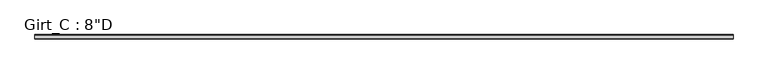
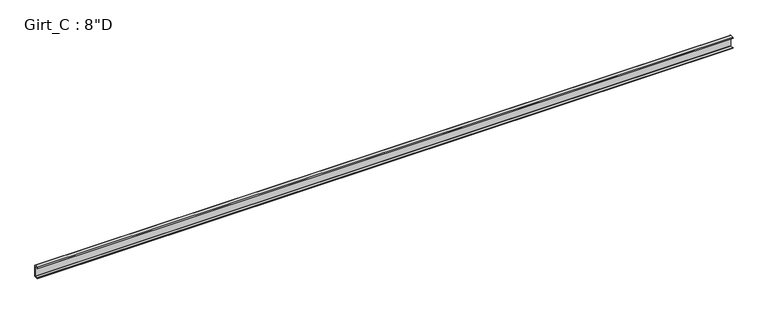
"""IFC4 building model written with IfcOpenShell, lengths in millimetres: beam geometry."""

from ifc_helpers import new_model, si_unit, point, frame, frame_2d, origin, place, context, project, spatial, polyline, circle_curve, trimmed, segment, composite_curve, outline, extrude, source, transform, mapped, element, save


def beam_6fe79ef6(model_context):
    return source(origin(), model_context, "Body", "SweptSolid", [
        extrude(outline(composite_curve([segment(polyline([(-63.5, 101.6), (-3.3734375, 101.6)]), True, "CONTINUOUS"), segment(trimmed(circle_curve(frame_2d((-3.3734375, 96.8375)), 4.7625), [point((-3.3734375, 101.6))], [point((1.3890625, 96.8375))], False, "CARTESIAN"), True, "CONTINUOUS"), segment(polyline([(1.3890625, 96.8375), (1.3890625, -96.8375)]), True, "CONTINUOUS"), segment(trimmed(circle_curve(frame_2d((-3.3734375, -96.8375)), 4.7625), [point((1.3890625, -96.8375))], [point((-3.3734375, -101.6))], False, "CARTESIAN"), True, "CONTINUOUS"), segment(polyline([(-3.3734375, -101.6), (-63.5, -101.6), (-75.745104, -87.0068534), (-73.6169367, -85.221109), (-62.204539, -98.821875), (-3.2694106, -98.821875)]), True, "CONTINUOUS"), segment(trimmed(circle_curve(frame_2d((-3.3748024, -96.8389339)), 1.9857399), [point((-3.2694106, -98.821875))], [point((-1.3890625, -96.8389339))], True, "CARTESIAN"), True, "CONTINUOUS"), segment(polyline([(-1.3890625, -96.8389339), (-1.3890625, 96.8381931)]), True, "CONTINUOUS"), segment(trimmed(circle_curve(frame_2d((-3.3741066, 96.8381931)), 1.9850441), [point((-1.3890625, 96.8381931))], [point((-3.3005807, 98.821875))], True, "CARTESIAN"), True, "CONTINUOUS"), segment(polyline([(-3.3005807, 98.821875), (-62.204539, 98.821875), (-73.6169367, 85.221109), (-75.745104, 87.0068534), (-63.5, 101.6)]), True, "CONTINUOUS")], self_intersect=False)), frame((-6007.1, 0.0, 0.0), z_axis=(1.0, 0.0, 0.0), x_axis=(0.0, 1.0, 0.0)), (0.0, 0.0, 1.0), 12014.2),
    ])


if __name__ == "__main__":
    model = new_model("IFC4")
    model_context = context("Model", 3, world=origin())
    ifc_project = project(units=[si_unit("LENGTHUNIT", "METRE", prefix="MILLI")], contexts=[model_context])
    site = spatial("IfcSite", under=ifc_project)
    building = spatial("IfcBuilding", under=site)
    placement = place(None, origin())
    beam_shape = beam_6fe79ef6(model_context)
    element("IfcBeam", 1, ObjectType="Girt_C : 8\"D", at=placement, inside=building, context=model_context, shape_type="MappedRepresentation", body=[
        mapped(beam_shape, transform((0.0, 0.0, 0.0), x_axis=(1.0, 0.0, 0.0), y_axis=(0.0, 1.0, 0.0), z_axis=(0.0, 0.0, 1.0))),
    ])
    save(model, "model.ifc")

# Revit data of these elements
# Type "Girt_C : 8\"D"
#   Web_Thickness = 0' - 0 7/64"
#   Length [instance default] = 10' - 0"
#   Leg_1 = 0' - 2 1/2"
#   Height = 0' - 8"
#   Structural Material [instance default] = none
# Element 1 (IfcBeam, "Girt_C : 8\"D")
#   Structural Material = Steel
#   Materials on its faces: "Steel"
# Materials
#   "Steel": class "Metal", colour RGB 118 118 114, transparency 0, Description = "Steel, mill finish", Cost = 0
